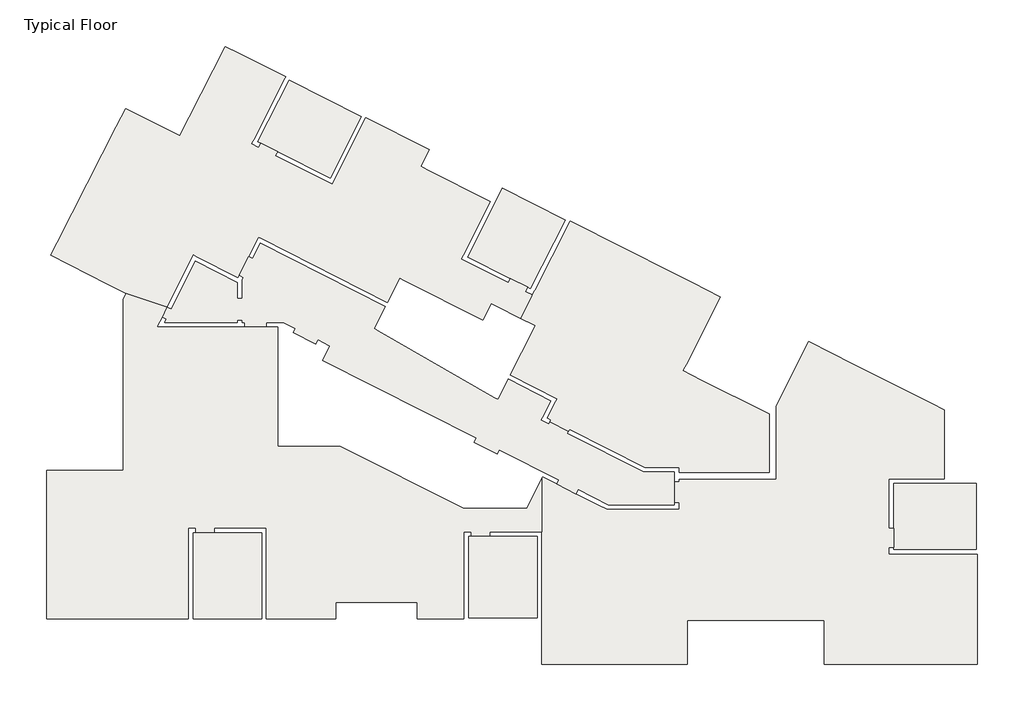
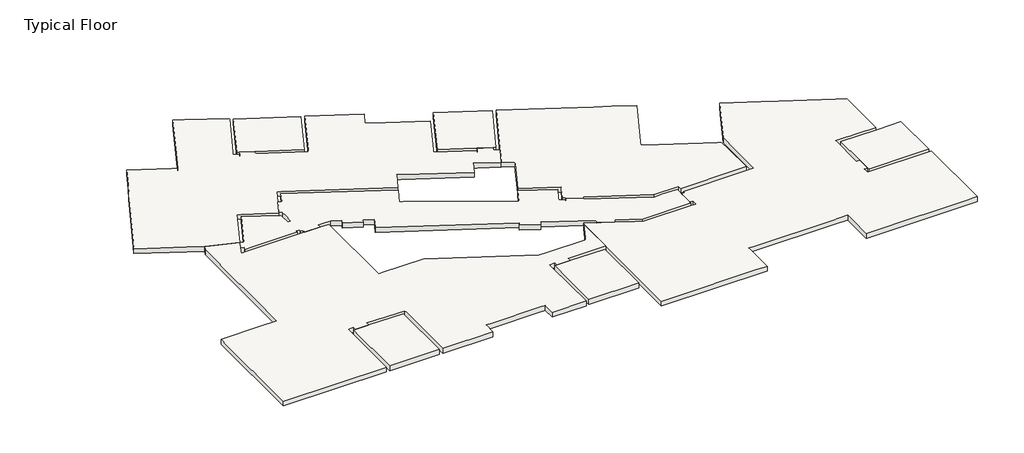
# One storey: 10 slabs.
"""IFC4 building model written with IfcOpenShell, lengths in millimetres."""

from ifc_helpers import new_model, si_unit, origin, place, context, project, spatial, faceted_brep, element, save

model = new_model("IFC4")

# Units and contexts
model_context = context("Model", 3, world=origin())
ifc_project = project(units=[si_unit("LENGTHUNIT", "METRE", prefix="MILLI")], contexts=[model_context])

# Site, building, storey
site = spatial("IfcSite", under=ifc_project)
building = spatial("IfcBuilding", under=site)
storey = spatial("IfcBuildingStorey", under=building, Name="Typical Floor", Elevation=3080.0)

# Slabs
placement = place(None, origin())
element("IfcSlab", 1, ObjectType="30", at=placement, inside=storey, context=model_context, shape_type="Brep", body=[
    faceted_brep([(-16793.6398388, -532.9875537, 2780.0), (-16673.4133533, -297.1586783, 2780.0), (-14950.1525065, -873.0331795, 2780.0), (-15159.2990357, -1291.3262379, 2780.0), (-15376.8855909, -1726.4993482, 2780.0), (-15153.2787931, -1726.4993482, 2780.0), (-11648.323755, -1726.4993482, 2780.0), (-10748.7939096, -1726.4993482, 2780.0), (-10246.1154665, -1726.4993482, 2780.0), (-10246.1154665, -6780.8119163, 2780.0), (-10046.1154665, -6780.8119163, 2780.0), (-7595.6314981, -6780.8119163, 2780.0), (-2368.5637573, -9419.7199019, 2780.0), (-1924.7869329, -9419.7199019, 2780.0), (311.4275518, -9419.7199019, 2780.0), (411.4275518, -9219.7199019, 2780.0), (945.0940817, -8152.386842, 2780.0), (945.0940817, -10417.0421397, 2780.0), (-1256.1083637, -10417.0421397, 2780.0), (-1256.1083637, -10617.0421397, 2780.0), (-2055.1025205, -10617.0421397, 2780.0), (-2055.1025205, -10417.0421397, 2780.0), (-2356.7095864, -10417.0421397, 2780.0), (-2356.7095864, -10617.0421397, 2780.0), (-2356.7095864, -14116.2328988, 2780.0), (-4337.2823123, -14116.2328988, 2780.0), (-4337.2823123, -13416.2328988, 2780.0), (-4637.2823123, -13416.2328988, 2780.0), (-7499.9037617, -13416.2328988, 2780.0), (-7799.9037617, -13416.2328988, 2780.0), (-7799.9037617, -14116.2328988, 2780.0), (-10738.2112055, -14116.2328988, 2780.0), (-10738.2112055, -10457.2302015, 2780.0), (-10738.2112055, -10257.2302015, 2780.0), (-12939.4136509, -10257.2302015, 2780.0), (-12939.4136509, -10457.2302015, 2780.0), (-13738.4078078, -10457.2302015, 2780.0), (-13738.4078078, -10257.2302015, 2780.0), (-14040.0148736, -10257.2302015, 2780.0), (-14040.0148736, -10457.2302015, 2780.0), (-14040.0148736, -14116.2328988, 2780.0), (-20057.3945771, -14116.2328988, 2780.0), (-20057.3945771, -7806.9823068, 2780.0), (-17693.6398388, -7806.9823068, 2780.0), (-16793.6398388, -7806.9823068, 2780.0), (-16793.6398388, -7506.9823068, 2780.0), (-16793.6398388, -4507.7754014, 2780.0), (-16793.6398388, -3607.7754014, 2780.0), (-16673.4133533, -297.1586783, 3080.0), (-16793.6398388, -532.9875537, 3080.0), (-16793.6398388, -3607.7754014, 3080.0), (-16793.6398388, -4507.7754014, 3080.0), (-16793.6398388, -7506.9823068, 3080.0), (-16793.6398388, -7806.9823068, 3080.0), (-17693.6398388, -7806.9823068, 3080.0), (-20057.3945771, -7806.9823068, 3080.0), (-20057.3945771, -8406.9823068, 3080.0), (-20057.3945771, -13520.1864188, 3080.0), (-20057.3945771, -14116.2328988, 3080.0), (-14040.0148736, -14116.2328988, 3080.0), (-14040.0148736, -10457.2302015, 3080.0), (-14040.0148736, -10257.2302015, 3080.0), (-13738.4078078, -10257.2302015, 3080.0), (-13738.4078078, -10457.2302015, 3080.0), (-12939.4136509, -10457.2302015, 3080.0), (-12939.4136509, -10257.2302015, 3080.0), (-10738.2112055, -10257.2302015, 3080.0), (-10738.2112055, -10457.2302015, 3080.0), (-10738.2112055, -14116.2328988, 3080.0), (-7799.9037617, -14116.2328988, 3080.0), (-7799.9037617, -13416.2328988, 3080.0), (-7499.9037617, -13416.2328988, 3080.0), (-4637.2823123, -13416.2328988, 3080.0), (-4337.2823123, -13416.2328988, 3080.0), (-4337.2823123, -14116.2328988, 3080.0), (-2356.7095864, -14116.2328988, 3080.0), (-2356.7095864, -10617.0421397, 3080.0), (-2356.7095864, -10417.0421397, 3080.0), (-2055.1025205, -10417.0421397, 3080.0), (-2055.1025205, -10617.0421397, 3080.0), (-1256.1083637, -10617.0421397, 3080.0), (-1256.1083637, -10417.0421397, 3080.0), (945.0940817, -10417.0421397, 3080.0), (945.0940817, -8152.386842, 3080.0), (411.4275518, -9219.7199019, 3080.0), (311.4275518, -9419.7199019, 3080.0), (-1924.7869329, -9419.7199019, 3080.0), (-2368.5637573, -9419.7199019, 3080.0), (-7595.6314981, -6780.8119163, 3080.0), (-10046.1154665, -6780.8119163, 3080.0), (-10246.1154665, -6780.8119163, 3080.0), (-10246.1154665, -1726.4993482, 3080.0), (-10748.7939096, -1726.4993482, 3080.0), (-11648.323755, -1726.4993482, 3080.0), (-15153.2787931, -1726.4993482, 3080.0), (-15376.8855909, -1726.4993482, 3080.0), (-15159.2990357, -1291.3262379, 3080.0), (-14950.1525065, -873.0331795, 3080.0)], [[[0, 1, 2, 3, 4, 5, 6, 7, 8, 9, 10, 11, 12, 13, 14, 15, 16, 17, 18, 19, 20, 21, 22, 23, 24, 25, 26, 27, 28, 29, 30, 31, 32, 33, 34, 35, 36, 37, 38, 39, 40, 41, 42, 43, 44, 45, 46, 47]], [[48, 49, 50, 51, 52, 53, 54, 55, 56, 57, 58, 59, 60, 61, 62, 63, 64, 65, 66, 67, 68, 69, 70, 71, 72, 73, 74, 75, 76, 77, 78, 79, 80, 81, 82, 83, 84, 85, 86, 87, 88, 89, 90, 91, 92, 93, 94, 95, 96, 97]], [[53, 44, 43, 42, 55, 54]], [[44, 53, 52, 51, 50, 49, 0, 47, 46, 45]], [[1, 0, 49, 48]], [[2, 1, 48, 97]], [[2, 97, 96, 95, 4, 3]], [[4, 95, 94, 93, 6, 5]], [[6, 93, 92, 91, 8, 7]], [[9, 8, 91, 90]], [[9, 90, 89, 88, 11, 10]], [[12, 11, 88, 87]], [[12, 87, 86, 85, 14, 13]], [[14, 85, 84, 83, 16, 15]], [[17, 16, 83, 82]], [[18, 17, 82, 81]], [[19, 18, 81, 80]], [[20, 19, 80, 79]], [[21, 20, 79, 78]], [[22, 21, 78, 77]], [[22, 77, 76, 75, 24, 23]], [[25, 24, 75, 74]], [[26, 25, 74, 73]], [[26, 73, 72, 71, 70, 29, 28, 27]], [[30, 29, 70, 69]], [[31, 30, 69, 68]], [[31, 68, 67, 66, 33, 32]], [[34, 33, 66, 65]], [[35, 34, 65, 64]], [[36, 35, 64, 63]], [[37, 36, 63, 62]], [[38, 37, 62, 61]], [[38, 61, 60, 59, 40, 39]], [[41, 40, 59, 58]], [[42, 41, 58, 57, 56, 55]]]),
])
element("IfcSlab", 2, ObjectType="30", at=placement, inside=storey, context=model_context, shape_type="Brep", body=[
    faceted_brep([(-10938.2112055, -10457.2302015, 2780.0), (-10938.2112055, -14116.2328988, 2780.0), (-13840.0148736, -14116.2328988, 2780.0), (-13840.0148736, -10457.2302015, 2780.0), (-13738.4078078, -10457.2302015, 2780.0), (-12939.4136509, -10457.2302015, 2780.0), (-10938.2112055, -14116.2328988, 3080.0), (-10938.2112055, -10457.2302015, 3080.0), (-12939.4136509, -10457.2302015, 3080.0), (-13738.4078078, -10457.2302015, 3080.0), (-13840.0148736, -10457.2302015, 3080.0), (-13840.0148736, -14116.2328988, 3080.0)], [[[0, 1, 2, 3, 4, 5]], [[6, 7, 8, 9, 10, 11]], [[1, 0, 7, 6]], [[2, 1, 6, 11]], [[3, 2, 11, 10]], [[3, 10, 9, 8, 7, 0, 5, 4]]]),
])
element("IfcSlab", 3, ObjectType="30", at=placement, inside=storey, context=model_context, shape_type="Brep", body=[
    faceted_brep([(745.0940817, -10617.0421397, 2780.0), (745.0940817, -14066.2328988, 2780.0), (-2156.7095864, -14066.2328988, 2780.0), (-2156.7095864, -10617.0421397, 2780.0), (-2055.1025205, -10617.0421397, 2780.0), (-1256.1083637, -10617.0421397, 2780.0), (745.0940817, -14066.2328988, 3080.0), (745.0940817, -10617.0421397, 3080.0), (-1256.1083637, -10617.0421397, 3080.0), (-2055.1025205, -10617.0421397, 3080.0), (-2156.7095864, -10617.0421397, 3080.0), (-2156.7095864, -14066.2328988, 3080.0)], [[[0, 1, 2, 3, 4, 5]], [[6, 7, 8, 9, 10, 11]], [[1, 0, 7, 6]], [[2, 1, 6, 11]], [[3, 2, 11, 10]], [[3, 10, 9, 8, 7, 0, 5, 4]]]),
])
element("IfcSlab", 4, ObjectType="30", at=placement, inside=storey, context=model_context, shape_type="Brep", body=[
    faceted_brep([(-11365.3254355, 6050.4914885, 2780.0), (-11061.2160035, 5898.43751, 2780.0), (-11060.9410199, 5898.98748, 2780.0), (-10971.4986478, 6077.8730917, 2780.0), (-10261.3883145, 5722.8196471, 2780.0), (-10350.8317224, 5543.9328312, 2780.0), (-10350.4815757, 5543.7577579, 2780.0), (-7938.3895863, 4337.7117632, 2780.0), (-7848.38183, 4516.3146828, 2780.0), (-6512.212519, 7167.6832976, 2780.0), (-3830.7495474, 5813.1866015, 2780.0), (-4191.4499427, 5099.1171197, 2780.0), (-3923.6738871, 4963.8544714, 2780.0), (-1236.2326264, 3606.3379414, 2780.0), (-2375.0336984, 1341.5313152, 2780.0), (-2464.8801865, 1162.8478502, 2780.0), (-483.5705934, 161.4417612, 2780.0), (-393.3538456, 339.9380873, 2780.0), (342.6939711, -32.0798789, 2780.0), (252.4772233, -210.576205, 2780.0), (555.5276046, -363.7458551, 2780.0), (54.7682985, -1356.8687143, 2780.0), (-1025.0324244, -812.4040937, 2780.0), (-1203.6158756, -722.3575055, 2780.0), (-1565.8606533, -1434.9049253, 2780.0), (-4895.2767918, 257.7032792, 2780.0), (-5073.5606377, 348.3392009, 2780.0), (-5598.1752698, -683.5950755, 2780.0), (-10896.1212839, 2009.7741272, 2780.0), (-11074.4066313, 2100.4108122, 2780.0), (-11488.3315473, 1277.8677098, 2780.0), (-11892.5037799, 474.7049399, 2780.0), (-11938.2560624, 383.7869427, 2780.0), (-13661.6245504, 1256.8091372, 2780.0), (-13840.040473, 1347.1908875, 2780.0), (-14950.1525065, -873.0331795, 2780.0), (-16673.4133533, -297.1586783, 2780.0), (-17475.2288855, 111.6100244, 2780.0), (-19872.740079, 1333.8706328, 2780.0), (-19600.2276105, 1868.414321, 2780.0), (-17692.9134653, 5609.6843751, 2780.0), (-17284.1447626, 6411.4999073, 2780.0), (-16701.0058274, 7555.3493571, 2780.0), (-16700.3132376, 7554.9985056, 2780.0), (-14670.4797396, 6526.7275889, 2780.0), (-14402.8595429, 6391.1568314, 2780.0), (-13996.1472702, 7194.0174215, 2780.0), (-12481.9034742, 10183.1740059, 2780.0), (-11946.0632398, 9912.5031689, 2780.0), (-11943.8088624, 9916.9661031, 2780.0), (-9919.3091434, 8894.3235346, 2780.0), (-9921.5753848, 8889.8665932, 2780.0), (-9944.2377986, 8845.2971792, 2780.0), (-11274.3950314, 6229.3212835, 2780.0), (-11365.0464358, 6051.0401879, 2780.0), (-11061.2160035, 5898.43751, 3080.0), (-11365.3254355, 6050.4914885, 3080.0), (-11365.0464358, 6051.0401879, 3080.0), (-11274.3950314, 6229.3212835, 3080.0), (-9944.2377986, 8845.2971792, 3080.0), (-9919.3091434, 8894.3235346, 3080.0), (-11943.8088624, 9916.9661031, 3080.0), (-11946.0632398, 9912.5031689, 3080.0), (-12481.9034742, 10183.1740059, 3080.0), (-12482.0593425, 10182.8663179, 3080.0), (-13996.1472702, 7194.0174215, 3080.0), (-14402.8595429, 6391.1568314, 3080.0), (-14670.4797396, 6526.7275889, 3080.0), (-14671.1406915, 6527.0624132, 3080.0), (-16700.3132376, 7554.9985056, 3080.0), (-16701.0058274, 7555.3493571, 3080.0), (-17284.1447626, 6411.4999073, 3080.0), (-17692.9134653, 5609.6843751, 3080.0), (-19600.2276105, 1868.414321, 3080.0), (-19872.740079, 1333.8706328, 3080.0), (-17475.2288855, 111.6100244, 3080.0), (-16673.4133533, -297.1586783, 3080.0), (-14950.1525065, -873.0331795, 3080.0), (-13840.040473, 1347.1908875, 3080.0), (-13661.6245504, 1256.8091372, 3080.0), (-11938.2560624, 383.7869427, 3080.0), (-11892.5037799, 474.7049399, 3080.0), (-11488.3315473, 1277.8677098, 3080.0), (-11074.4066313, 2100.4108122, 3080.0), (-10896.1212839, 2009.7741272, 3080.0), (-5598.1752698, -683.5950755, 3080.0), (-5073.5606377, 348.3392009, 3080.0), (-4895.2767918, 257.7032792, 3080.0), (-1565.8606533, -1434.9049253, 3080.0), (-1203.6158756, -722.3575055, 3080.0), (-1025.0324244, -812.4040937, 3080.0), (54.7682985, -1356.8687143, 3080.0), (555.5276046, -363.7458551, 3080.0), (252.4772233, -210.576205, 3080.0), (342.6939711, -32.0798789, 3080.0), (-393.3538456, 339.9380873, 3080.0), (-483.5705934, 161.4417612, 3080.0), (-2464.8801865, 1162.8478502, 3080.0), (-2375.0336984, 1341.5313152, 3080.0), (-1236.2326264, 3606.3379414, 3080.0), (-3923.6738871, 4963.8544714, 3080.0), (-4191.4499427, 5099.1171197, 3080.0), (-3830.7495474, 5813.1866015, 3080.0), (-6512.212519, 7167.6832976, 3080.0), (-7848.38183, 4516.3146828, 3080.0), (-7938.3895863, 4337.7117632, 3080.0), (-10350.4815757, 5543.7577579, 3080.0), (-10350.8317224, 5543.9328312, 3080.0), (-10261.3883145, 5722.8196471, 3080.0), (-10971.4986478, 6077.8730917, 3080.0), (-11060.9410199, 5898.98748, 3080.0)], [[[0, 1, 2, 3, 4, 5, 6, 7, 8, 9, 10, 11, 12, 13, 14, 15, 16, 17, 18, 19, 20, 21, 22, 23, 24, 25, 26, 27, 28, 29, 30, 31, 32, 33, 34, 35, 36, 37, 38, 39, 40, 41, 42, 43, 44, 45, 46, 47, 48, 49, 50, 51, 52, 53, 54]], [[55, 56, 57, 58, 59, 60, 61, 62, 63, 64, 65, 66, 67, 68, 69, 70, 71, 72, 73, 74, 75, 76, 77, 78, 79, 80, 81, 82, 83, 84, 85, 86, 87, 88, 89, 90, 91, 92, 93, 94, 95, 96, 97, 98, 99, 100, 101, 102, 103, 104, 105, 106, 107, 108, 109, 110]], [[66, 45, 44, 43, 42, 70, 69, 68, 67]], [[45, 66, 65, 64, 63, 47, 46]], [[60, 50, 49, 61]], [[50, 60, 59, 58, 57, 56, 0, 54, 53, 52, 51]], [[1, 0, 56, 55]], [[1, 55, 110, 109, 3, 2]], [[4, 3, 109, 108]], [[5, 4, 108, 107]], [[5, 107, 106, 105, 7, 6]], [[7, 105, 104, 103, 9, 8]], [[10, 9, 103, 102]], [[11, 10, 102, 101]], [[11, 101, 100, 99, 13, 12]], [[13, 99, 98, 97, 15, 14]], [[16, 15, 97, 96]], [[17, 16, 96, 95]], [[18, 17, 95, 94]], [[19, 18, 94, 93]], [[20, 19, 93, 92]], [[21, 20, 92, 91]], [[21, 91, 90, 89, 23, 22]], [[24, 23, 89, 88]], [[24, 88, 87, 86, 26, 25]], [[27, 26, 86, 85]], [[27, 85, 84, 83, 29, 28]], [[29, 83, 82, 81, 80, 32, 31, 30]], [[32, 80, 79, 78, 34, 33]], [[35, 34, 78, 77]], [[36, 35, 77, 76]], [[36, 76, 75, 74, 38, 37]], [[38, 74, 73, 72, 71, 70, 42, 41, 40, 39]], [[48, 62, 61, 49]], [[62, 48, 47, 63]]]),
])
element("IfcSlab", 5, ObjectType="30", at=placement, inside=storey, context=model_context, shape_type="Brep", body=[
    faceted_brep([(1942.7642171, 2824.3146799, 2780.0), (467.2492575, -95.0334036, 2780.0), (343.0939217, -32.2820245, 2780.0), (342.6939711, -32.0798789, 2780.0), (-393.3542192, 339.9382762, 2780.0), (-2196.5369883, 1251.3143734, 2780.0), (-727.390856, 4173.099378, 2780.0), (467.2492575, -95.0334036, 3080.0), (1942.7642171, 2824.3146799, 3080.0), (-727.390856, 4173.099378, 3080.0), (-2196.5369883, 1251.3143734, 3080.0), (-393.3542192, 339.9382762, 3080.0), (342.6939711, -32.0798789, 3080.0), (343.0939217, -32.2820245, 3080.0)], [[[0, 1, 2, 3, 4, 5, 6]], [[7, 8, 9, 10, 11, 12, 13]], [[1, 0, 8, 7]], [[1, 7, 13, 12, 11, 10, 5, 4, 3, 2]], [[6, 5, 10, 9]], [[0, 6, 9, 8]]]),
])
element("IfcSlab", 6, ObjectType="30", at=placement, inside=storey, context=model_context, shape_type="Brep", body=[
    faceted_brep([(-11095.5055118, 6139.8765236, 2780.0), (-9765.7197974, 8755.1217618, 2780.0), (-6713.2317343, 7213.2078736, 2780.0), (-8027.2639377, 4605.7557366, 2780.0), (-10261.0388566, 5722.6431961, 2780.0), (-10261.3890033, 5722.8182694, 2780.0), (-10971.4984738, 6077.8730046, 2780.0), (-9765.7197974, 8755.1217618, 3080.0), (-11095.5055118, 6139.8765236, 3080.0), (-10971.4984738, 6077.8730046, 3080.0), (-10261.3890033, 5722.8182694, 3080.0), (-10261.0388566, 5722.6431961, 3080.0), (-8027.2639377, 4605.7557366, 3080.0), (-6713.2317343, 7213.2078736, 3080.0)], [[[0, 1, 2, 3, 4, 5, 6]], [[7, 8, 9, 10, 11, 12, 13]], [[1, 0, 8, 7]], [[2, 1, 7, 13]], [[3, 2, 13, 12]], [[3, 12, 11, 10, 9, 8, 0, 6, 5, 4]]]),
])
element("IfcSlab", 7, ObjectType="30", at=placement, inside=storey, context=model_context, shape_type="Brep", body=[
    faceted_brep([(6770.8726693, -9468.8187486, 2780.0), (6770.8726693, -9167.2116828, 2780.0), (6570.8726693, -9167.2116828, 2780.0), (6570.8726693, -8294.9401934, 2780.0), (6770.8726693, -8294.9401934, 2780.0), (6770.8726693, -8186.8724338, 2780.0), (9983.8347444, -8186.8724338, 2780.0), (10883.8347444, -8186.8724338, 2780.0), (10883.8347444, -7886.8724338, 2780.0), (10883.8347444, -5941.560553, 2780.0), (10883.8347444, -5068.3107696, 2780.0), (11994.586414, -2869.3836839, 2780.0), (12265.1117105, -2333.8315725, 2780.0), (14139.6409418, -3280.7190282, 2780.0), (14942.9691088, -3686.5069729, 2780.0), (17519.0395063, -4987.7663524, 2780.0), (18024.1024442, -5242.8905469, 2780.0), (18024.1024442, -8167.1461487, 2780.0), (15870.9267875, -8167.1461487, 2780.0), (15670.9267875, -8167.1461487, 2780.0), (15670.9267875, -10267.8129055, 2780.0), (15870.9267875, -10267.8129055, 2780.0), (15870.9267875, -11066.8070624, 2780.0), (15670.9267875, -11066.8070624, 2780.0), (15670.9267875, -11368.4141282, 2780.0), (15870.9267875, -11368.4141282, 2780.0), (19424.1024442, -11368.4141282, 2780.0), (19424.1024442, -16035.9823018, 2780.0), (12920.9090644, -16035.9823018, 2780.0), (12920.9090644, -14474.4460263, 2780.0), (12920.9090644, -14174.4460263, 2780.0), (12020.9090644, -14174.4460263, 2780.0), (7425.6343679, -14174.4460263, 2780.0), (7125.6343679, -14174.4460263, 2780.0), (7125.6343679, -15074.4460263, 2780.0), (7125.6343679, -16035.9823018, 2780.0), (945.0940817, -16035.9823018, 2780.0), (945.0940817, -10417.0421397, 2780.0), (945.0940817, -8152.386842, 2780.0), (979.8740908, -8083.6419805, 2780.0), (1576.7028432, -8385.594867, 2780.0), (2397.1569943, -8800.6862953, 2780.0), (3322.4500467, -9268.8187486, 2780.0), (3717.7625467, -9468.8187486, 2780.0), (6570.8726693, -9468.8187486, 2780.0), (6770.8726693, -9167.2116828, 3080.0), (6770.8726693, -9468.8187486, 3080.0), (6570.8726693, -9468.8187486, 3080.0), (3717.7625467, -9468.8187486, 3080.0), (3322.4500467, -9268.8187486, 3080.0), (2397.1569943, -8800.6862953, 3080.0), (1576.7028432, -8385.594867, 3080.0), (979.8740908, -8083.6419805, 3080.0), (945.0940817, -8152.386842, 3080.0), (945.0940817, -10417.0421397, 3080.0), (945.0940817, -10617.0421397, 3080.0), (945.0940817, -14066.2328988, 3080.0), (945.0940817, -14416.2328988, 3080.0), (945.0940817, -16035.9823018, 3080.0), (1545.0940817, -16035.9823018, 3080.0), (6525.6343679, -16035.9823018, 3080.0), (7125.6343679, -16035.9823018, 3080.0), (7125.6343679, -15074.4460263, 3080.0), (7125.6343679, -14174.4460263, 3080.0), (7425.6343679, -14174.4460263, 3080.0), (12020.9090644, -14174.4460263, 3080.0), (12920.9090644, -14174.4460263, 3080.0), (12920.9090644, -14474.4460263, 3080.0), (12920.9090644, -16035.9823018, 3080.0), (13520.9090644, -16035.9823018, 3080.0), (18824.1024442, -16035.9823018, 3080.0), (19424.1024442, -16035.9823018, 3080.0), (19424.1024442, -11368.4141282, 3080.0), (15870.9267875, -11368.4141282, 3080.0), (15670.9267875, -11368.4141282, 3080.0), (15670.9267875, -11066.8070624, 3080.0), (15870.9267875, -11066.8070624, 3080.0), (15870.9267875, -10267.8129055, 3080.0), (15670.9267875, -10267.8129055, 3080.0), (15670.9267875, -8167.1461487, 3080.0), (15870.9267875, -8167.1461487, 3080.0), (18024.1024442, -8167.1461487, 3080.0), (18024.1024442, -5242.8905469, 3080.0), (17519.0395063, -4987.7663524, 3080.0), (14942.9691088, -3686.5069729, 3080.0), (14139.6409418, -3280.7190282, 3080.0), (12265.1117105, -2333.8315725, 3080.0), (11994.586414, -2869.3836839, 3080.0), (10883.8347444, -5068.3107696, 3080.0), (10883.8347444, -5941.560553, 3080.0), (10883.8347444, -7886.8724338, 3080.0), (10883.8347444, -8186.8724338, 3080.0), (9983.8347444, -8186.8724338, 3080.0), (6770.8726693, -8186.8724338, 3080.0), (6770.8726693, -8294.9401934, 3080.0), (6570.8726693, -8294.9401934, 3080.0), (6570.8726693, -9167.2116828, 3080.0)], [[[0, 1, 2, 3, 4, 5, 6, 7, 8, 9, 10, 11, 12, 13, 14, 15, 16, 17, 18, 19, 20, 21, 22, 23, 24, 25, 26, 27, 28, 29, 30, 31, 32, 33, 34, 35, 36, 37, 38, 39, 40, 41, 42, 43, 44]], [[45, 46, 47, 48, 49, 50, 51, 52, 53, 54, 55, 56, 57, 58, 59, 60, 61, 62, 63, 64, 65, 66, 67, 68, 69, 70, 71, 72, 73, 74, 75, 76, 77, 78, 79, 80, 81, 82, 83, 84, 85, 86, 87, 88, 89, 90, 91, 92, 93, 94, 95, 96]], [[46, 0, 44, 43, 48, 47]], [[1, 0, 46, 45]], [[2, 1, 45, 96]], [[3, 2, 96, 95]], [[4, 3, 95, 94]], [[5, 4, 94, 93]], [[5, 93, 92, 91, 7, 6]], [[7, 91, 90, 89, 88, 10, 9, 8]], [[10, 88, 87, 86, 12, 11]], [[12, 86, 85, 84, 83, 82, 16, 15, 14, 13]], [[17, 16, 82, 81]], [[17, 81, 80, 79, 19, 18]], [[20, 19, 79, 78]], [[21, 20, 78, 77]], [[22, 21, 77, 76]], [[23, 22, 76, 75]], [[24, 23, 75, 74]], [[24, 74, 73, 72, 26, 25]], [[27, 26, 72, 71]], [[28, 27, 71, 70, 69, 68]], [[28, 68, 67, 66, 30, 29]], [[30, 66, 65, 64, 63, 33, 32, 31]], [[33, 63, 62, 61, 35, 34]], [[36, 35, 61, 60, 59, 58]], [[38, 37, 36, 58, 57, 56, 55, 54, 53]], [[48, 43, 42, 41, 40, 39, 52, 51, 50, 49]], [[39, 38, 53, 52]]]),
])
element("IfcSlab", 8, ObjectType="30", at=placement, inside=storey, context=model_context, shape_type="Brep", body=[
    faceted_brep([(19374.1024442, -8367.1461487, 2780.0), (19374.1024442, -11168.4141282, 2780.0), (15870.9267875, -11168.4141282, 2780.0), (15870.9267875, -11066.8070624, 2780.0), (15870.9267875, -10267.8129055, 2780.0), (15870.9267875, -8367.1461487, 2780.0), (19374.1024442, -11168.4141282, 3080.0), (19374.1024442, -8367.1461487, 3080.0), (18025.5784419, -8367.1461487, 3080.0), (15870.9267875, -8367.1461487, 3080.0), (15870.9267875, -10267.8129055, 3080.0), (15870.9267875, -11066.8070624, 3080.0), (15870.9267875, -11168.4141282, 3080.0)], [[[0, 1, 2, 3, 4, 5]], [[6, 7, 8, 9, 10, 11, 12]], [[1, 0, 7, 6]], [[2, 1, 6, 12]], [[2, 12, 11, 10, 9, 5, 4, 3]], [[0, 5, 9, 8, 7]]]),
])
element("IfcSlab", 9, ObjectType="30", at=placement, inside=storey, context=model_context, shape_type="Brep", body=[
    faceted_brep([(10598.8347444, -7886.8724338, 2780.0), (10583.8347444, -7886.8724338, 2780.0), (6770.8726693, -7886.8724338, 2780.0), (6770.8726693, -7674.9401934, 2780.0), (6570.8726693, -7674.9401934, 2780.0), (5313.1307352, -7674.9401934, 2780.0), (2125.3800884, -6062.6233374, 2780.0), (2077.6094062, -6157.0719084, 2780.0), (1275.5029536, -5748.919163, 2780.0), (1322.2831712, -5656.4288636, 2780.0), (1179.5082357, -5584.2154251, 2780.0), (1595.97634, -4765.1614866, 2780.0), (-382.0351871, -3757.2575237, 2780.0), (671.5014835, -1667.8412216, 2780.0), (54.7682985, -1356.8687143, 2780.0), (555.5276046, -363.7458551, 2780.0), (548.7903843, -360.3406864, 2780.0), (638.8365216, -181.7581293, 2780.0), (645.7455836, -185.2501513, 2780.0), (2143.8361829, 2778.7634578, 2780.0), (6570.712081, 542.6002731, 2780.0), (7374.040248, 136.8123284, 2780.0), (8515.9105496, -439.9845796, 2780.0), (7067.4162986, -3307.5321414, 2780.0), (6932.1536504, -3575.3081971, 2780.0), (7735.4818174, -3981.0961419, 2780.0), (10583.8347444, -5419.8945403, 2780.0), (10583.8347444, -5941.560553, 2780.0), (10598.8347444, -5941.560553, 2780.0), (6770.8726693, -7886.8724338, 3080.0), (9983.8347444, -7886.8724338, 3080.0), (10598.8347444, -7886.8724338, 3080.0), (10598.8347444, -5941.560553, 3080.0), (10583.8347444, -5941.560553, 3080.0), (10583.8347444, -5419.8945403, 3080.0), (10413.5787556, -5333.8925419, 3080.0), (7735.4818174, -3981.0961419, 3080.0), (6932.1536504, -3575.3081971, 3080.0), (7067.4162986, -3307.5321414, 3080.0), (8515.9105496, -439.9845796, 3080.0), (7374.040248, 136.8123284, 3080.0), (6570.712081, 542.6002731, 3080.0), (2143.8361829, 2778.7634578, 3080.0), (645.7455836, -185.2501513, 3080.0), (638.8365216, -181.7581293, 3080.0), (548.7903843, -360.3406864, 3080.0), (555.5276046, -363.7458551, 3080.0), (54.7682985, -1356.8687143, 3080.0), (671.5014835, -1667.8412216, 3080.0), (581.4556142, -1846.4238115, 3080.0), (-382.0351871, -3757.2575237, 3080.0), (1595.97634, -4765.1614866, 3080.0), (1505.3269714, -4943.4385782, 3080.0), (1179.5082357, -5584.2154251, 3080.0), (1322.2831712, -5656.4288636, 3080.0), (1275.5029536, -5748.919163, 3080.0), (2077.6094062, -6157.0719084, 3080.0), (2125.3800884, -6062.6233374, 3080.0), (5313.1307352, -7674.9401934, 3080.0), (6570.8726693, -7674.9401934, 3080.0), (6770.8726693, -7674.9401934, 3080.0)], [[[0, 1, 2, 3, 4, 5, 6, 7, 8, 9, 10, 11, 12, 13, 14, 15, 16, 17, 18, 19, 20, 21, 22, 23, 24, 25, 26, 27, 28]], [[29, 30, 31, 32, 33, 34, 35, 36, 37, 38, 39, 40, 41, 42, 43, 44, 45, 46, 47, 48, 49, 50, 51, 52, 53, 54, 55, 56, 57, 58, 59, 60]], [[39, 22, 21, 20, 19, 42, 41, 40]], [[22, 39, 38, 37, 24, 23]], [[24, 37, 36, 35, 34, 26, 25]], [[31, 0, 28, 32]], [[2, 1, 0, 31, 30, 29]], [[3, 2, 29, 60]], [[3, 60, 59, 58, 5, 4]], [[6, 5, 58, 57]], [[7, 6, 57, 56]], [[7, 56, 55, 8]], [[44, 17, 16, 45]], [[12, 50, 49, 48, 13]], [[11, 51, 50, 12]], [[51, 11, 10, 53, 52]], [[18, 43, 42, 19]], [[43, 18, 17, 44]], [[15, 46, 45, 16]], [[46, 15, 14, 47]], [[27, 33, 32, 28]], [[33, 27, 26, 34]], [[9, 54, 53, 10]], [[54, 9, 8, 55]], [[13, 48, 47, 14]]]),
])
element("IfcSlab", 10, ObjectType="30", at=placement, inside=storey, context=model_context, shape_type="Brep", body=[
    faceted_brep([(-13751.0685018, 1077.9212344, 2780.0), (-11960.5135249, 170.863779, 2780.0), (-11960.5135249, -518.38158, 2780.0), (-11760.5135249, -518.38158, 2780.0), (-11760.5135249, 69.5479895, 2780.0), (-11760.5135249, 293.7463151, 2780.0), (-11759.841961, 293.406115, 2780.0), (-11713.8494576, 384.8014744, 2780.0), (-11892.5037799, 474.7049399, 2780.0), (-11488.3315473, 1277.8677098, 2780.0), (-11309.677225, 1187.9642443, 2780.0), (-10986.0255065, 1831.1183002, 2780.0), (-5688.8111915, -861.8789214, 2780.0), (-6161.1916976, -1791.0669498, 2780.0), (-5982.9078517, -1881.7028715, 2780.0), (-1082.8838189, -4702.990676, 2780.0), (-904.301229, -4793.0365453, 2780.0), (-472.0818656, -3935.8417186, 2780.0), (1327.1276693, -4852.636386, 2780.0), (1001.0372857, -5493.9474736, 2780.0), (910.387743, -5672.2249076, 2780.0), (1232.0154262, -5834.8994051, 2780.0), (1275.5029536, -5748.919163, 2780.0), (2077.6096629, -6157.072039, 2780.0), (2035.1126004, -6241.094009, 2780.0), (5265.429403, -7874.9401934, 2780.0), (5708.5555718, -7874.9401934, 2780.0), (6570.8726693, -7874.9401934, 2780.0), (6570.8726693, -8294.9401934, 2780.0), (6570.8726693, -9167.2116828, 2780.0), (6570.8726693, -9268.8187486, 2780.0), (3765.4759744, -9268.8187486, 2780.0), (2487.4451637, -8622.2260855, 2780.0), (2397.1569943, -8800.6862953, 2780.0), (1576.7028432, -8385.594867, 2780.0), (1666.9910125, -8207.1346573, 2780.0), (-860.136602, -6928.58788, 2780.0), (-950.4247713, -7107.0480897, 2780.0), (-1927.470094, -6613.7824899, 2780.0), (-1838.1570872, -6436.8740342, 2780.0), (-8353.2474072, -3147.7022221, 2780.0), (-8129.2939322, -2699.7952722, 2780.0), (-8039.8512131, -2520.909834, 2780.0), (-8558.6189839, -2261.5259486, 2780.0), (-8648.061703, -2440.4113868, 2780.0), (-9601.9030088, -1963.4907339, 2780.0), (-9512.4602897, -1784.6052957, 2780.0), (-10028.6721847, -1526.4993482, 2780.0), (-10475.8857802, -1526.4993482, 2780.0), (-10748.7939096, -1526.4993482, 2780.0), (-10748.7939096, -1726.4993482, 2780.0), (-11648.323755, -1726.4993482, 2780.0), (-11648.323755, -1526.4993482, 2780.0), (-11760.5135249, -1526.4993482, 2780.0), (-11760.5135249, -1425.9636596, 2780.0), (-11960.5135249, -1425.9636596, 2780.0), (-11960.5135249, -1526.4993482, 2780.0), (-15053.2787931, -1526.4993482, 2780.0), (-14980.4135975, -1380.768957, 2780.0), (-15159.2990357, -1291.3262379, 2780.0), (-14950.1525065, -873.0331795, 2780.0), (-14771.2670683, -962.4758986, 2780.0), (-11960.5135249, 170.863779, 3080.0), (-13751.0685018, 1077.9212344, 3080.0), (-14771.2670683, -962.4758986, 3080.0), (-14950.1525065, -873.0331795, 3080.0), (-15159.2990357, -1291.3262379, 3080.0), (-14980.4135975, -1380.768957, 3080.0), (-15053.2787931, -1526.4993482, 3080.0), (-11960.5135249, -1526.4993482, 3080.0), (-11960.5135249, -1425.9636596, 3080.0), (-11760.5135249, -1425.9636596, 3080.0), (-11760.5135249, -1526.4993482, 3080.0), (-11648.323755, -1526.4993482, 3080.0), (-11648.323755, -1726.4993482, 3080.0), (-10748.7939096, -1726.4993482, 3080.0), (-10748.7939096, -1526.4993482, 3080.0), (-10475.8857802, -1526.4993482, 3080.0), (-10028.6721847, -1526.4993482, 3080.0), (-9512.4602897, -1784.6052957, 3080.0), (-9601.9030088, -1963.4907339, 3080.0), (-8648.061703, -2440.4113868, 3080.0), (-8558.6189839, -2261.5259486, 3080.0), (-8039.8512131, -2520.909834, 3080.0), (-8129.2939322, -2699.7952722, 3080.0), (-8353.2474072, -3147.7022221, 3080.0), (-1838.1570872, -6436.8740342, 3080.0), (-1927.470094, -6613.7824899, 3080.0), (-950.4247713, -7107.0480897, 3080.0), (-860.136602, -6928.58788, 3080.0), (1666.9910125, -8207.1346573, 3080.0), (1576.7028432, -8385.594867, 3080.0), (2397.1569943, -8800.6862953, 3080.0), (2487.4451637, -8622.2260855, 3080.0), (3765.4759744, -9268.8187486, 3080.0), (6570.8726693, -9268.8187486, 3080.0), (6570.8726693, -9167.2116828, 3080.0), (6570.8726693, -8294.9401934, 3080.0), (6570.8726693, -7874.9401934, 3080.0), (5708.5555718, -7874.9401934, 3080.0), (5265.429403, -7874.9401934, 3080.0), (2035.1126004, -6241.094009, 3080.0), (2077.6096629, -6157.072039, 3080.0), (1275.5029536, -5748.919163, 3080.0), (1232.0154262, -5834.8994051, 3080.0), (910.387743, -5672.2249076, 3080.0), (1001.0372857, -5493.9474736, 3080.0), (1327.1276693, -4852.636386, 3080.0), (-472.0818656, -3935.8417186, 3080.0), (-904.301229, -4793.0365453, 3080.0), (-1082.8838189, -4702.990676, 3080.0), (-5982.9078517, -1881.7028715, 3080.0), (-6161.1916976, -1791.0669498, 3080.0), (-5688.8111915, -861.8789214, 3080.0), (-10986.0255065, 1831.1183002, 3080.0), (-11309.677225, 1187.9642443, 3080.0), (-11488.3315473, 1277.8677098, 3080.0), (-11892.5037799, 474.7049399, 3080.0), (-11713.8494576, 384.8014744, 3080.0), (-11759.841961, 293.406115, 3080.0), (-11760.5135249, 293.7463151, 3080.0), (-11760.5135249, 69.5479895, 3080.0), (-11760.5135249, -518.38158, 3080.0), (-11960.5135249, -518.38158, 3080.0)], [[[0, 1, 2, 3, 4, 5, 6, 7, 8, 9, 10, 11, 12, 13, 14, 15, 16, 17, 18, 19, 20, 21, 22, 23, 24, 25, 26, 27, 28, 29, 30, 31, 32, 33, 34, 35, 36, 37, 38, 39, 40, 41, 42, 43, 44, 45, 46, 47, 48, 49, 50, 51, 52, 53, 54, 55, 56, 57, 58, 59, 60, 61]], [[62, 63, 64, 65, 66, 67, 68, 69, 70, 71, 72, 73, 74, 75, 76, 77, 78, 79, 80, 81, 82, 83, 84, 85, 86, 87, 88, 89, 90, 91, 92, 93, 94, 95, 96, 97, 98, 99, 100, 101, 102, 103, 104, 105, 106, 107, 108, 109, 110, 111, 112, 113, 114, 115, 116, 117, 118, 119, 120, 121, 122, 123]], [[1, 0, 63, 62]], [[2, 1, 62, 123]], [[3, 2, 123, 122]], [[3, 122, 121, 120, 5, 4]], [[8, 7, 118, 117]], [[9, 8, 117, 116]], [[10, 9, 116, 115]], [[11, 10, 115, 114]], [[12, 11, 114, 113]], [[13, 12, 113, 112]], [[14, 13, 112, 111]], [[15, 14, 111, 110]], [[15, 110, 109, 16]], [[105, 20, 19, 18, 107, 106]], [[20, 105, 104, 21]], [[101, 24, 23, 102]], [[25, 24, 101, 100]], [[25, 100, 99, 98, 27, 26]], [[27, 98, 97, 96, 95, 30, 29, 28]], [[31, 30, 95, 94]], [[32, 31, 94, 93]], [[33, 32, 93, 92]], [[34, 33, 92, 91]], [[35, 34, 91, 90]], [[36, 35, 90, 89]], [[37, 36, 89, 88]], [[38, 37, 88, 87]], [[39, 38, 87, 86]], [[40, 39, 86, 85]], [[40, 85, 84, 83, 42, 41]], [[43, 42, 83, 82]], [[44, 43, 82, 81]], [[45, 44, 81, 80]], [[46, 45, 80, 79]], [[47, 46, 79, 78]], [[47, 78, 77, 76, 49, 48]], [[50, 49, 76, 75]], [[51, 50, 75, 74]], [[52, 51, 74, 73]], [[53, 52, 73, 72]], [[54, 53, 72, 71]], [[55, 54, 71, 70]], [[56, 55, 70, 69]], [[57, 56, 69, 68]], [[0, 61, 64, 63]], [[6, 119, 118, 7]], [[119, 6, 5, 120]], [[16, 109, 108, 17]], [[21, 104, 103, 22]], [[58, 57, 68, 67]], [[59, 58, 67, 66]], [[60, 59, 66, 65]], [[61, 60, 65, 64]], [[23, 22, 103, 102]], [[18, 17, 108, 107]]]),
])

save(model, "model.ifc")

# Revit data of these elements
# Type "30"
#   Function = 0
#   Layers, outside or top first: 30 cm "Concrete" (function 1)
# Element 1 (IfcSlab, "30")
#   Mark = "S1"
#   SOFiSTiK_AMG_Comments = ""
#   built-in parameter 1001955 = 1.5708 (stored number, unit not read)
#   Height Offset From Level = 0 cm
#   built-in parameter 1001954 = 1
#   SOFiSTiK_AMG_Scheduled = yes
#   SOFiSTiK_AMG_Adjusted = yes
#   Phase Created = New Construction
#   Materials on its faces: "Concrete"
# Element 2 (IfcSlab, "30")
#   Mark = "S2"
#   SOFiSTiK_AMG_Comments = ""
#   Height Offset From Level = 0 cm
#   built-in parameter 1001954 = 1
#   SOFiSTiK_AMG_Scheduled = yes
#   SOFiSTiK_AMG_Adjusted = yes
#   Phase Created = New Construction
#   Materials on its faces: "Concrete"
# Element 3 (IfcSlab, "30")
#   Mark = "S3"
#   SOFiSTiK_AMG_Comments = ""
#   Height Offset From Level = 0 cm
#   built-in parameter 1001954 = 1
#   SOFiSTiK_AMG_Scheduled = yes
#   SOFiSTiK_AMG_Adjusted = yes
#   Phase Created = New Construction
#   Materials on its faces: "Concrete"
# Element 4 (IfcSlab, "30")
#   Mark = "S4"
#   SOFiSTiK_AMG_Comments = ""
#   built-in parameter 1001955 = 1.09934 (stored number, unit not read)
#   Height Offset From Level = 0 cm
#   built-in parameter 1001954 = 1
#   SOFiSTiK_AMG_Scheduled = yes
#   SOFiSTiK_AMG_Adjusted = yes
#   Phase Created = New Construction
#   Materials on its faces: "Concrete"
# Element 5 (IfcSlab, "30")
#   Mark = "S5"
#   SOFiSTiK_AMG_Comments = ""
#   built-in parameter 1001955 = -0.467746 (stored number, unit not read)
#   Height Offset From Level = 0 cm
#   built-in parameter 1001954 = 1
#   SOFiSTiK_AMG_Scheduled = yes
#   SOFiSTiK_AMG_Adjusted = yes
#   Phase Created = New Construction
#   Materials on its faces: "Concrete"
# Element 6 (IfcSlab, "30")
#   Mark = "S6"
#   SOFiSTiK_AMG_Comments = ""
#   built-in parameter 1001955 = -2.0412 (stored number, unit not read)
#   Height Offset From Level = 0 cm
#   built-in parameter 1001954 = 1
#   SOFiSTiK_AMG_Scheduled = yes
#   SOFiSTiK_AMG_Adjusted = yes
#   Phase Created = New Construction
#   Materials on its faces: "Concrete"
# Element 7 (IfcSlab, "30")
#   Mark = "S7"
#   SOFiSTiK_AMG_Comments = ""
#   built-in parameter 1001955 = -0.468379 (stored number, unit not read)
#   Height Offset From Level = 0 cm
#   built-in parameter 1001954 = 1
#   SOFiSTiK_AMG_Scheduled = yes
#   SOFiSTiK_AMG_Adjusted = yes
#   Phase Created = New Construction
#   Materials on its faces: "Concrete"
# Element 8 (IfcSlab, "30")
#   Mark = "S8"
#   SOFiSTiK_AMG_Comments = ""
#   Height Offset From Level = 0 cm
#   built-in parameter 1001954 = 1
#   SOFiSTiK_AMG_Scheduled = yes
#   SOFiSTiK_AMG_Adjusted = yes
#   Phase Created = New Construction
#   Materials on its faces: "Concrete"
# Element 9 (IfcSlab, "30")
#   Mark = "S9"
#   SOFiSTiK_AMG_Comments = ""
#   built-in parameter 1001955 = 1.10377 (stored number, unit not read)
#   Height Offset From Level = 0 cm
#   built-in parameter 1001954 = 1
#   SOFiSTiK_AMG_Scheduled = yes
#   SOFiSTiK_AMG_Adjusted = yes
#   Phase Created = New Construction
#   Materials on its faces: "Concrete"
# Element 10 (IfcSlab, "30")
#   Mark = "S10"
#   SOFiSTiK_AMG_Comments = ""
#   built-in parameter 1001955 = 1.10715 (stored number, unit not read)
#   Height Offset From Level = 0 cm
#   built-in parameter 1001954 = 1
#   SOFiSTiK_AMG_Scheduled = yes
#   SOFiSTiK_AMG_Adjusted = no
#   Phase Created = New Construction
#   Materials on its faces: "Concrete"
# Materials
#   "Concrete": class "Concrete", colour RGB 192 192 192, transparency 0, Keynote = "01000", Description = "Cast-in-place concrete", Cost = 0
